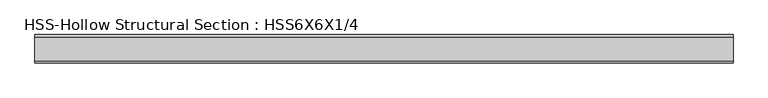
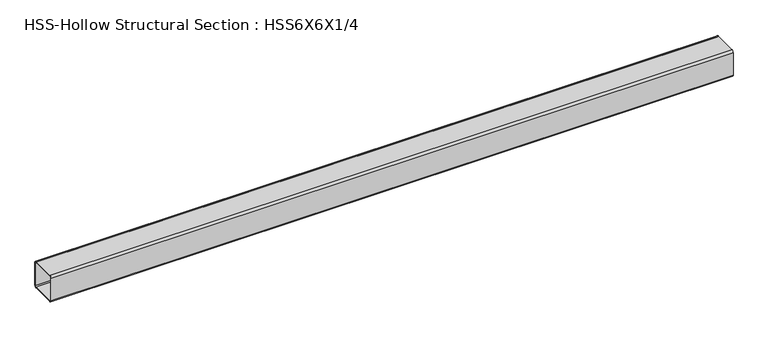
"""IFC4 building model written with IfcOpenShell, lengths in millimetres: beam geometry, HSS-Hollow Structural Section : HSS6X6X1/4."""

from ifc_helpers import new_model, si_unit, point, frame, frame_2d, origin, place, context, project, spatial, polyline, circle_curve, trimmed, segment, composite_curve, outline, extrude, source, transform, mapped, element, save


def hss_hollow_structural_section_hss6x6x1_4_7611db10(model_context):
    return source(origin(), model_context, "Body", "SweptSolid", [
        extrude(outline(composite_curve([segment(polyline([(76.2, 64.3636), (76.2, -64.3636)]), True, "CONTINUOUS"), segment(trimmed(circle_curve(frame_2d((64.3636, -64.3636)), 11.8364), [point((76.2, -64.3636))], [point((64.3636, -76.2))], False, "CARTESIAN"), True, "CONTINUOUS"), segment(polyline([(64.3636, -76.2), (-64.3636, -76.2)]), True, "CONTINUOUS"), segment(trimmed(circle_curve(frame_2d((-64.3636, -64.3636)), 11.8364), [point((-64.3636, -76.2))], [point((-76.2, -64.3636))], False, "CARTESIAN"), True, "CONTINUOUS"), segment(polyline([(-76.2, -64.3636), (-76.2, 64.3636)]), True, "CONTINUOUS"), segment(trimmed(circle_curve(frame_2d((-64.3636, 64.3636)), 11.8364), [point((-76.2, 64.3636))], [point((-64.3636, 76.2))], False, "CARTESIAN"), True, "CONTINUOUS"), segment(polyline([(-64.3636, 76.2), (64.3636, 76.2)]), True, "CONTINUOUS"), segment(trimmed(circle_curve(frame_2d((64.3636, 64.3636)), 11.8364), [point((64.3636, 76.2))], [point((76.2, 64.3636))], False, "CARTESIAN"), True, "CONTINUOUS")], self_intersect=False), holes=[composite_curve([segment(trimmed(circle_curve(frame_2d((-64.3636, 64.3636)), 5.9182), [point((-64.3636, 70.2818))], [point((-70.2818, 64.3636))], True, "CARTESIAN"), True, "CONTINUOUS"), segment(polyline([(-70.2818, 64.3636), (-70.2818, -64.3636)]), True, "CONTINUOUS"), segment(trimmed(circle_curve(frame_2d((-64.3636, -64.3636)), 5.9182), [point((-70.2818, -64.3636))], [point((-64.3636, -70.2818))], True, "CARTESIAN"), True, "CONTINUOUS"), segment(polyline([(-64.3636, -70.2818), (64.3636, -70.2818)]), True, "CONTINUOUS"), segment(trimmed(circle_curve(frame_2d((64.3636, -64.3636)), 5.9182), [point((64.3636, -70.2818))], [point((70.2818, -64.3636))], True, "CARTESIAN"), True, "CONTINUOUS"), segment(polyline([(70.2818, -64.3636), (70.2818, 64.3636)]), True, "CONTINUOUS"), segment(trimmed(circle_curve(frame_2d((64.3636, 64.3636)), 5.9182), [point((70.2818, 64.3636))], [point((64.3636, 70.2818))], True, "CARTESIAN"), True, "CONTINUOUS"), segment(polyline([(64.3636, 70.2818), (-64.3636, 70.2818)]), True, "CONTINUOUS")], self_intersect=False)]), frame((-1866.9677845, 0.0, 0.0), z_axis=(1.0, 0.0, 0.0), x_axis=(0.0, 1.0, 0.0)), (0.0, 0.0, 1.0), 3733.8677845),
    ])


if __name__ == "__main__":
    model = new_model("IFC4")
    model_context = context("Model", 3, world=origin())
    ifc_project = project(units=[si_unit("LENGTHUNIT", "METRE", prefix="MILLI")], contexts=[model_context])
    site = spatial("IfcSite", under=ifc_project)
    building = spatial("IfcBuilding", under=site)
    placement = place(None, origin())
    hss_hollow_structural_section_hss6x6x1_4_shape = hss_hollow_structural_section_hss6x6x1_4_7611db10(model_context)
    element("IfcBeam", 1, ObjectType="HSS-Hollow Structural Section : HSS6X6X1/4", at=placement, inside=building, context=model_context, shape_type="MappedRepresentation", body=[
        mapped(hss_hollow_structural_section_hss6x6x1_4_shape, transform((0.0, 0.0, 0.0), x_axis=(1.0, 0.0, 0.0), y_axis=(0.0, 1.0, 0.0), z_axis=(0.0, 0.0, 1.0))),
    ])
    save(model, "model.ifc")

# Revit data of these elements
# Type "HSS-Hollow Structural Section : HSS6X6X1/4"
#   Assembly Code = "B10"
#   Shape = "Square"
#   W = 19
#   Ht = 0' - 6"
#   Length [instance default] = 5' - 0"
#   b = 0' - 6"
#   kr = 0' - 0.466"
#   t = 0' - 0.233"
#   A = 0.0363889 SF
#   Structural Material [instance default] = Steel ASTM A500, Grade B, Rectangular and Square
# Element 1 (IfcBeam, "HSS-Hollow Structural Section : HSS6X6X1/4")
#   Materials on its faces: "Steel ASTM A500, Grade B, Rectangular and Square"
# Materials
#   "Steel ASTM A500, Grade B, Rectangular and Square": class "Metal", colour RGB 199 199 199, transparency 0, Description = "Carbon steel", Cost = 0
